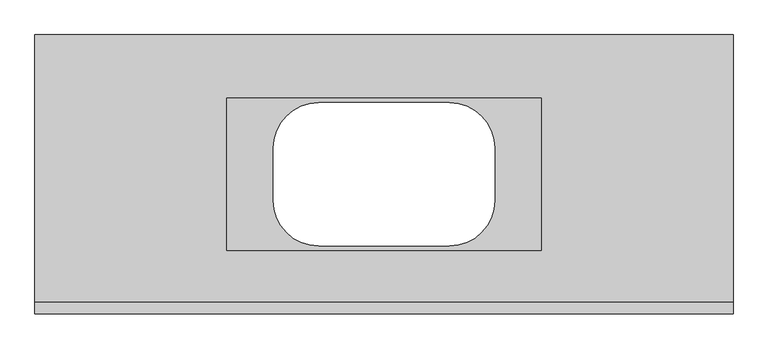
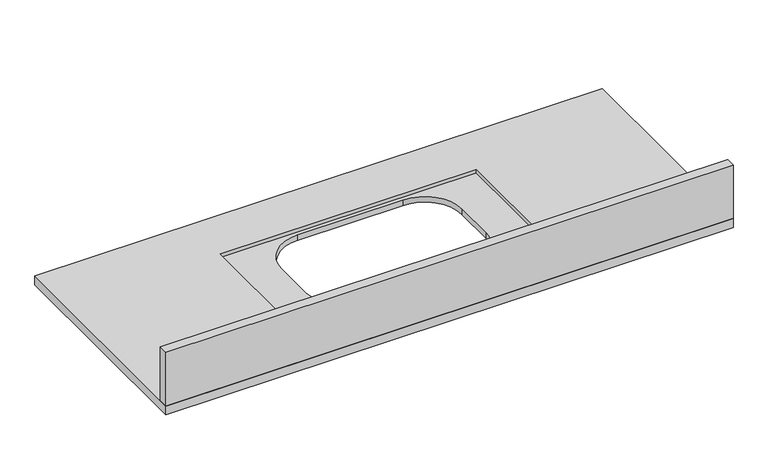
"""IFC4 building model written with IfcOpenShell, lengths in millimetres: furniture geometry, CC_BANCADA COZINHA RETA_1 CUBA QUADRADA : CC_BANCADA COZINHA RETA_1 CUBA QUADRADA."""

from ifc_helpers import new_model, si_unit, frame, origin, place, context, project, spatial, polyline, circle_curve, outline, extrude, source, transform, mapped, element, save
from ifc_brep_helpers import plane_surface, revolved_surface, advanced_brep


def furniture_e0bd580f(model_context):
    return source(origin(), model_context, "Body", "SolidModel", [
        advanced_brep(
        [(794.7003264, 0.0, 900.0), (794.7003264, 600.0, 900.0), (-705.2996736, 600.0, 900.0), (-705.2996736, 0.0, 900.0), (-293.2996736, 136.0, 900.0), (-293.2996736, 464.0, 900.0), (382.7003264, 464.0, 900.0), (382.7003264, 136.0, 900.0), (-705.2996736, 0.0, 875.0), (-705.2996736, 600.0, 875.0), (794.7003264, 600.0, 875.0), (794.7003264, 0.0, 875.0), (-193.2996736, 356.0, 875.0), (-193.2996736, 244.0, 875.0), (-95.2996736, 146.0, 875.0), (184.7003264, 146.0, 875.0), (282.7003264, 244.0, 875.0), (282.7003264, 356.0, 875.0), (184.7003264, 454.0, 875.0), (-95.2996736, 454.0, 875.0), (382.7003264, 136.0, 890.0), (382.7003264, 464.0, 890.0), (-293.2996736, 464.0, 890.0), (-293.2996736, 136.0, 890.0), (-95.2996736, 454.0, 890.0), (184.7003264, 454.0, 890.0), (282.7003264, 356.0, 890.0), (282.7003264, 244.0, 890.0), (184.7003264, 146.0, 890.0), (-95.2996736, 146.0, 890.0), (-193.2996736, 244.0, 890.0), (-193.2996736, 356.0, 890.0)],
        [
            (0, 1),
            (1, 2),
            (2, 3),
            (3, 0),
            (4, 5),
            (5, 6),
            (6, 7),
            (7, 4),
            (8, 9),
            (9, 10),
            (10, 11),
            (11, 8),
            (12, 13),
            (13, 14, circle_curve(frame((-95.2996736, 244.0, 875.0), z_axis=(0.0, 0.0, 1.0), x_axis=(1.0, 0.0, 0.0)), 98.0)),
            (14, 15),
            (15, 16, circle_curve(frame((184.7003264, 244.0, 875.0), z_axis=(0.0, 0.0, 1.0), x_axis=(1.0, 0.0, 0.0)), 98.0)),
            (16, 17),
            (17, 18, circle_curve(frame((184.7003264, 356.0, 875.0), z_axis=(0.0, 0.0, 1.0), x_axis=(1.0, 0.0, 0.0)), 98.0)),
            (18, 19),
            (19, 12, circle_curve(frame((-95.2996736, 356.0, 875.0), z_axis=(0.0, 0.0, 1.0), x_axis=(1.0, 0.0, 0.0)), 98.0)),
            (3, 8),
            (11, 0),
            (2, 9),
            (1, 10),
            (20, 21),
            (21, 22),
            (22, 23),
            (23, 20),
            (24, 25),
            (25, 26, circle_curve(frame((184.7003264, 356.0, 890.0), z_axis=(0.0, 0.0, -1.0), x_axis=(1.0, 0.0, 0.0)), 98.0)),
            (26, 27),
            (27, 28, circle_curve(frame((184.7003264, 244.0, 890.0), z_axis=(0.0, 0.0, -1.0), x_axis=(1.0, 0.0, 0.0)), 98.0)),
            (28, 29),
            (29, 30, circle_curve(frame((-95.2996736, 244.0, 890.0), z_axis=(0.0, 0.0, -1.0), x_axis=(1.0, 0.0, 0.0)), 98.0)),
            (30, 31),
            (31, 24, circle_curve(frame((-95.2996736, 356.0, 890.0), z_axis=(0.0, 0.0, -1.0), x_axis=(1.0, 0.0, 0.0)), 98.0)),
            (23, 4),
            (7, 20),
            (22, 5),
            (21, 6),
            (19, 24),
            (31, 12),
            (15, 28),
            (27, 16),
            (14, 29),
            (13, 30),
            (17, 26),
            (25, 18),
        ],
        [
            plane_surface(frame((-705.2996736, 0.0, 900.0), z_axis=(0.0, 0.0, 1.0), x_axis=(-1.0, 0.0, 0.0))),
            plane_surface(frame((-705.2996736, 0.0, 875.0), z_axis=(0.0, 0.0, -1.0), x_axis=(1.0, 0.0, 0.0))),
            plane_surface(frame((794.7003264, 0.0, 900.0), z_axis=(0.0, -1.0, 0.0), x_axis=(0.0, 0.0, -1.0))),
            plane_surface(frame((-705.2996736, 0.0, 900.0), z_axis=(-1.0, 0.0, 0.0), x_axis=(0.0, 0.0, -1.0))),
            plane_surface(frame((-705.2996736, 600.0, 900.0), z_axis=(0.0, 1.0, 0.0), x_axis=(0.0, 0.0, -1.0))),
            plane_surface(frame((794.7003264, 600.0, 900.0), z_axis=(1.0, 0.0, 0.0), x_axis=(0.0, 0.0, -1.0))),
            plane_surface(frame((-293.2996736, 136.0, 890.0), z_axis=(0.0, 0.0, 1.0), x_axis=(1.0, 0.0, 0.0))),
            plane_surface(frame((382.7003264, 136.0, 900.0), z_axis=(0.0, 1.0, 0.0), x_axis=(0.0, 0.0, -1.0))),
            plane_surface(frame((-293.2996736, 136.0, 900.0), z_axis=(1.0, 0.0, 0.0), x_axis=(0.0, 0.0, -1.0))),
            plane_surface(frame((-293.2996736, 464.0, 900.0), z_axis=(0.0, -1.0, 0.0), x_axis=(0.0, 0.0, -1.0))),
            plane_surface(frame((382.7003264, 464.0, 900.0), z_axis=(-1.0, 0.0, 0.0), x_axis=(0.0, 0.0, -1.0))),
            revolved_surface(polyline([(2.7003263999999945, 356.0, 890.0), (2.7003263999999945, 356.0, 875.0)]), (-95.2996736, 356.0, 875.0), (0.0, 0.0, 1.0)),
            revolved_surface(polyline([(282.7003264, 244.0, 890.0), (282.7003264, 244.0, 875.0)]), (184.7003264, 244.0, 875.0), (0.0, 0.0, 1.0)),
            plane_surface(frame((184.7003264, 146.0, 900.0), z_axis=(0.0, 1.0, 0.0), x_axis=(0.0, 0.0, -1.0))),
            revolved_surface(polyline([(2.7003263999999945, 244.0, 890.0), (2.7003263999999945, 244.0, 875.0)]), (-95.2996736, 244.0, 875.0), (0.0, 0.0, 1.0)),
            plane_surface(frame((-193.2996736, 244.0, 900.0), z_axis=(1.0, 0.0, 0.0), x_axis=(0.0, 0.0, -1.0))),
            revolved_surface(polyline([(282.7003264, 356.0, 890.0), (282.7003264, 356.0, 875.0)]), (184.7003264, 356.0, 875.0), (0.0, 0.0, 1.0)),
            plane_surface(frame((282.7003264, 356.0, 900.0), z_axis=(-1.0, 0.0, 0.0), x_axis=(0.0, 0.0, -1.0))),
            plane_surface(frame((-95.2996736, 454.0, 900.0), z_axis=(0.0, -1.0, 0.0), x_axis=(0.0, 0.0, -1.0))),
        ],
        [
            (0, [[1, 2, 3, 4], [5, 6, 7, 8]]),
            (1, [[9, 10, 11, 12], [13, 14, 15, 16, 17, 18, 19, 20]]),
            (2, [[21, -12, 22, -4]]),
            (3, [[23, -9, -21, -3]]),
            (4, [[24, -10, -23, -2]]),
            (5, [[-22, -11, -24, -1]]),
            (6, [[25, 26, 27, 28], [29, 30, 31, 32, 33, 34, 35, 36]]),
            (7, [[37, -8, 38, -28]]),
            (8, [[39, -5, -37, -27]]),
            (9, [[40, -6, -39, -26]]),
            (10, [[-38, -7, -40, -25]]),
            (11, [[41, -36, 42, -20]]),
            (12, [[43, -32, 44, -16]]),
            (13, [[45, -33, -43, -15]]),
            (14, [[46, -34, -45, -14]]),
            (15, [[-42, -35, -46, -13]]),
            (16, [[47, -30, 48, -18]]),
            (17, [[-44, -31, -47, -17]]),
            (18, [[-48, -29, -41, -19]]),
        ],
    ),
        extrude(outline(polyline([(794.7003264, 0.0), (-705.2996736, 0.0), (-705.2996736, 25.0), (794.7003264, 25.0), (794.7003264, 0.0)])), frame((0.0, 0.0, 900.0), z_axis=(0.0, 0.0, 1.0), x_axis=(1.0, 0.0, 0.0)), (0.0, 0.0, 1.0), 150.0),
    ])


if __name__ == "__main__":
    model = new_model("IFC4")
    model_context = context("Model", 3, world=origin())
    ifc_project = project(units=[si_unit("LENGTHUNIT", "METRE", prefix="MILLI")], contexts=[model_context])
    site = spatial("IfcSite", under=ifc_project)
    building = spatial("IfcBuilding", under=site)
    placement = place(None, origin())
    furniture_shape = furniture_e0bd580f(model_context)
    element("IfcFurniture", 1, ObjectType="CC_BANCADA COZINHA RETA_1 CUBA QUADRADA : CC_BANCADA COZINHA RETA_1 CUBA QUADRADA", at=placement, inside=building, context=model_context, shape_type="MappedRepresentation", body=[
        mapped(furniture_shape, transform((0.0, 0.0, 0.0), x_axis=(1.0, 0.0, 0.0), y_axis=(0.0, 1.0, 0.0), z_axis=(0.0, 0.0, 1.0))),
    ])
    save(model, "model.ifc")

# Revit data of these elements
# Type "CC_BANCADA COZINHA RETA_1 CUBA QUADRADA : CC_BANCADA COZINHA RETA_1 CUBA QUADRADA"
#   Site = "www.construir.arq.br"
#   Empresa = "Cursos Construir"
#   Criado Por = "Roberto Netto"
#   Profunidade Área Molhada [instance default] = 0.01 m
#   Depth = 0.60 m
#   Espessura Frontão [instance default] = 0.025 m
#   Espessura Bancada [instance default] = 0.025 m
#   Espaçamento Posterior Área Molhada [instance default] = 0.01 m
#   Espaçamento Lateral Esquerda Cuba [instance default] = 0.75 m
#   Espaçamento Frontal Área Molhada [instance default] = 0.01 m
#   Espaçamento Frontal Cuba [instance default] = 0.30 m
#   Espaçamento Esquerdo Área Molhada [instance default] = 0.10 m
#   Espaçamento Direito Área Molhada [instance default] = 0.10 m
#   Height = 0.90 m
#   Width = 1.50 m
#   Altura Frontão [instance default] = 0.15 m
#   ----ÁREA MOLHADA---- [instance default] = 0.00 m
#   ----FRONTÃO---- [instance default] = 0.00 m
#   ----CUBA---- [instance default] = 0.00 m
#   ----BANCADA---- [instance default] = 0.00 m
#   Frontão Posterior [instance default] = yes
#   Frontão Esquerda [instance default] = yes
#   Frontão Direita [instance default] = yes
#   Cuba Centralizada [instance default] = yes
#   Material Frontão [instance default] = .BANCADA
#   Material Bancada [instance default] = .BANCADA
#   Default Elevation = 0
# Element 1 (IfcFurniture, "CC_BANCADA COZINHA RETA_1 CUBA QUADRADA : CC_BANCADA COZINHA RETA_1 CUBA QUADRADA")
#   Frontão Esquerda = no
#   Frontão Direita = no
#   Materials on its faces: ".BANCADA"
# Materials
#   ".BANCADA": class "Genérico", colour RGB 239 239 230, transparency 0, Cost = 0
